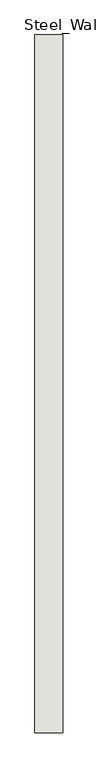
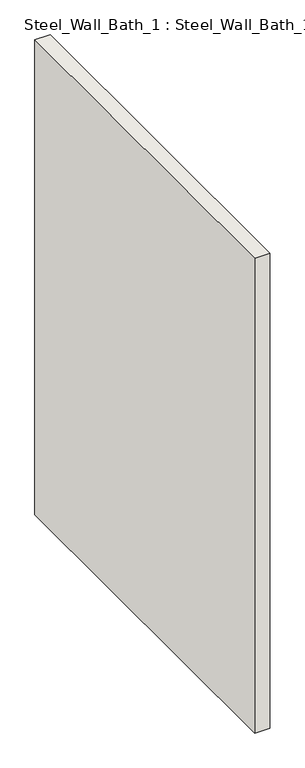
"""IFC4 building model written with IfcOpenShell, lengths in millimetres: wall geometry, Steel_Wall_Bath_1 : Steel_Wall_Bath_1."""

import ifcopenshell
import ifcopenshell.guid

model = None  # the IFC model being written
_history = None  # IfcOwnerHistory: only IFC2X3 demands one
_inside = {}  # id of a spatial element -> (the spatial element, [elements in it])
_under = {}  # id of a project, library or spatial element -> (it, [spatial elements below it])
_declared = {}  # id of a project -> (the project, [libraries it declares])
_typed = {}  # id of a type object -> (the type object, [elements of that type])
_made_of = {}  # id of a material, layer set ... -> (it, [elements and type objects made of it])


def new_model(schema):
    """Start an empty IFC model of exactly this schema.

    Asked for "IFC4X3", IfcOpenShell would pick the latest addendum, in which some entities
    have other attributes; the version numbers below select the first issue.
    IFC2X3 requires an IfcOwnerHistory on every rooted entity: one is made here for all.
    """
    global model, _history
    if schema == "IFC4X3":
        model = ifcopenshell.file(schema_version=(4, 3, 0, 0))
    else:
        model = ifcopenshell.file(schema=schema)
    _inside.clear()
    _under.clear()
    _declared.clear()
    _typed.clear()
    _made_of.clear()
    _history = None
    if model.schema == "IFC2X3":
        org = make("IfcOrganization", Name="unknown")
        user = make(
            "IfcPersonAndOrganization",
            ThePerson=make("IfcPerson", FamilyName="unknown"),
            TheOrganization=org,
        )
        app = make(
            "IfcApplication",
            ApplicationDeveloper=org,
            Version="unknown",
            ApplicationFullName="unknown",
            ApplicationIdentifier="unknown",
        )
        _history = make(
            "IfcOwnerHistory",
            OwningUser=user,
            OwningApplication=app,
            ChangeAction="ADDED",
            CreationDate=0,
        )
    return model


def make(cls, **values):
    """One entity of the class cls with the attributes given. An attribute that is None is left unset."""
    return model.create_entity(
        cls, **{name: value for name, value in values.items() if value is not None}
    )


def rooted(cls, **values):
    """An entity with a GlobalId (a new one), such as an element, a storey or a relation."""
    return make(cls, GlobalId=ifcopenshell.guid.new(), OwnerHistory=_history, **values)


def si_unit(unit_type, name, prefix=None):
    """IfcSIUnit, for example si_unit("LENGTHUNIT", "METRE", prefix="MILLI")."""
    return make("IfcSIUnit", UnitType=unit_type, Prefix=prefix, Name=name)


def assignment(units):
    """IfcUnitAssignment: the units of a project."""
    return None if units is None else make("IfcUnitAssignment", Units=units)


def point(xyz):
    """IfcCartesianPoint."""
    return None if xyz is None else make("IfcCartesianPoint", Coordinates=xyz)


def direction(xyz):
    """IfcDirection."""
    return None if xyz is None else make("IfcDirection", DirectionRatios=xyz)


def frame(location, z_axis=None, x_axis=None):
    """IfcAxis2Placement3D, a coordinate frame: its origin and axes. An axis left out is left unset."""
    return make(
        "IfcAxis2Placement3D",
        Location=point(location),
        Axis=direction(z_axis),
        RefDirection=direction(x_axis),
    )


def origin():
    """The frame at (0, 0, 0) with its axes left unset."""
    return frame((0.0, 0.0, 0.0))


def place(relative_to, where):
    """IfcLocalPlacement: puts the frame where relative to a parent placement (None: the world)."""
    return make(
        "IfcLocalPlacement", PlacementRelTo=relative_to, RelativePlacement=where
    )


def context(
    kind, dimensions, precision=None, world=None, true_north=None, identifier=None
):
    """IfcGeometricRepresentationContext, for example the 3D "Model" context."""
    return make(
        "IfcGeometricRepresentationContext",
        ContextIdentifier=identifier,
        ContextType=kind,
        CoordinateSpaceDimension=dimensions,
        Precision=precision,
        WorldCoordinateSystem=world,
        TrueNorth=true_north,
    )


def project(units=None, contexts=None):
    """IfcProject with its units and contexts."""
    return rooted(
        "IfcProject",
        Name="project",
        RepresentationContexts=contexts,
        UnitsInContext=assignment(units),
    )


def spatial(cls, under=None, at=None, **own):
    """A site, building, storey or space (cls), placed at a placement, below another one or the project."""
    s = rooted(cls, ObjectPlacement=at, **own)
    if under is not None:
        _under.setdefault(under.id(), (under, []))[1].append(s)
    return s


def polyline(points):
    """IfcPolyline through the points."""
    return make("IfcPolyline", Points=[point(p) for p in points])


def outline(outer, holes=None, kind="AREA"):
    """IfcArbitraryClosedProfileDef: a profile drawn as a closed curve; with holes, ...WithVoids."""
    if holes is None:
        return make("IfcArbitraryClosedProfileDef", ProfileType=kind, OuterCurve=outer)
    return make(
        "IfcArbitraryProfileDefWithVoids",
        ProfileType=kind,
        OuterCurve=outer,
        InnerCurves=holes,
    )


def extrude(swept, where, along, depth):
    """IfcExtrudedAreaSolid: the profile swept, set in the frame where, extruded along a direction by depth."""
    return make(
        "IfcExtrudedAreaSolid",
        SweptArea=swept,
        Position=where,
        ExtrudedDirection=direction(along),
        Depth=depth,
    )


def shape(context_of_items, identifier, shape_type, items):
    """IfcShapeRepresentation: the items that make up one representation, for example the "Body"."""
    return make(
        "IfcShapeRepresentation",
        ContextOfItems=context_of_items,
        RepresentationIdentifier=identifier,
        RepresentationType=shape_type,
        Items=items,
    )


def source(mapping_origin, context_of_items, identifier, shape_type, items):
    """IfcRepresentationMap: a shape defined once, which mapped items show again and again."""
    return make(
        "IfcRepresentationMap",
        MappingOrigin=mapping_origin,
        MappedRepresentation=shape(context_of_items, identifier, shape_type, items),
    )


def transform(
    local_origin,
    x_axis=None,
    y_axis=None,
    z_axis=None,
    scale=None,
    scale2=None,
    scale3=None,
    uniform=True,
):
    """IfcCartesianTransformationOperator3D, or its non-uniform kind. x_axis, y_axis, z_axis: its Axis1, 2, 3."""
    if uniform:
        return make(
            "IfcCartesianTransformationOperator3D",
            Axis1=direction(x_axis),
            Axis2=direction(y_axis),
            LocalOrigin=point(local_origin),
            Scale=scale,
            Axis3=direction(z_axis),
        )
    return make(
        "IfcCartesianTransformationOperator3DnonUniform",
        Axis1=direction(x_axis),
        Axis2=direction(y_axis),
        LocalOrigin=point(local_origin),
        Scale=scale,
        Axis3=direction(z_axis),
        Scale2=scale2,
        Scale3=scale3,
    )


def mapped(mapping_source, mapping_target):
    """IfcMappedItem: shows the shape of a source again, moved by a transform."""
    return make(
        "IfcMappedItem", MappingSource=mapping_source, MappingTarget=mapping_target
    )


def made_of(thing, what):
    """Note that an element or type object is made of a material, layer set ...; save() writes the relation."""
    if what is not None:
        _made_of.setdefault(what.id(), (what, []))[1].append(thing)
    return thing


def element(
    cls,
    number,
    at=None,
    inside=None,
    cuts=None,
    type_object=None,
    material=None,
    context=None,
    identifier="Body",
    shape_type=None,
    held_by="IfcProductDefinitionShape",
    body=None,
    shapes=None,
    **own,
):
    """One element of the class cls, such as IfcWall. Its Tag is "e" and its number.

    at: its placement. inside: the storey or other place that contains it. cuts: it is an
    opening in that element (IfcRelVoidsElement). A single representation is given by context,
    identifier, shape_type and body (its items); several are given by shapes. held_by: the class
    of the entity that holds the representations. save() writes the other relations.
    """
    e = rooted(cls, Tag="e%d" % number, ObjectPlacement=at, **own)
    if body is not None:
        shapes = [shape(context, identifier, shape_type, body)]
    if shapes is not None:
        e.Representation = make(held_by, Representations=shapes)
    if inside is not None:
        _inside.setdefault(inside.id(), (inside, []))[1].append(e)
    if cuts is not None:
        rooted(
            "IfcRelVoidsElement", RelatingBuildingElement=cuts, RelatedOpeningElement=e
        )
    if type_object is not None:
        _typed.setdefault(type_object.id(), (type_object, []))[1].append(e)
    return made_of(e, material)


def aggregate(whole, parts):
    """IfcRelAggregates: a whole, such as a stair, and the parts it consists of."""
    return rooted("IfcRelAggregates", RelatingObject=whole, RelatedObjects=parts)


def save(model, path):
    """Write the relations noted so far, then the file.

    IfcRelAggregates (storeys below a building ...), IfcRelContainedInSpatialStructure (elements
    in a storey), IfcRelDefinesByType, IfcRelAssociatesMaterial and IfcRelDeclares: one each for
    every whole, place, type object, material and project.
    """
    for whole, parts in _under.values():
        aggregate(whole, parts)
    for where, things in _inside.values():
        rooted(
            "IfcRelContainedInSpatialStructure",
            RelatedElements=things,
            RelatingStructure=where,
        )
    for kind, things in _typed.values():
        rooted("IfcRelDefinesByType", RelatedObjects=things, RelatingType=kind)
    for what, things in _made_of.values():
        rooted("IfcRelAssociatesMaterial", RelatedObjects=things, RelatingMaterial=what)
    for by, libraries in _declared.values():
        rooted("IfcRelDeclares", RelatingContext=by, RelatedDefinitions=libraries)
    model.write(path)


def steel_wall_bath_1_steel_wall_bath_1_50d80b11(model_context):
    return source(origin(), model_context, "Body", "SweptSolid", [
        extrude(outline(polyline([(4175.0, 14705.0), (4175.0, 12205.0), (4075.0, 12205.0), (4075.0, 14705.0), (4175.0, 14705.0)])), frame((0.0, 0.0, 250.0), z_axis=(0.0, 0.0, 1.0), x_axis=(1.0, 0.0, 0.0)), (0.0, 0.0, 1.0), 3300.0),
    ])


if __name__ == "__main__":
    model = new_model("IFC4")
    model_context = context("Model", 3, world=origin())
    ifc_project = project(units=[si_unit("LENGTHUNIT", "METRE", prefix="MILLI")], contexts=[model_context])
    site = spatial("IfcSite", under=ifc_project)
    building = spatial("IfcBuilding", under=site)
    placement = place(None, origin())
    steel_wall_bath_1_steel_wall_bath_1_shape = steel_wall_bath_1_steel_wall_bath_1_50d80b11(model_context)
    element("IfcWall", 1, ObjectType="Steel_Wall_Bath_1 : Steel_Wall_Bath_1", at=placement, inside=building, context=model_context, shape_type="MappedRepresentation", body=[
        mapped(steel_wall_bath_1_steel_wall_bath_1_shape, transform((0.0, 0.0, 0.0), x_axis=(1.0, 0.0, 0.0), y_axis=(0.0, 1.0, 0.0), z_axis=(0.0, 0.0, 1.0))),
    ])
    save(model, "model.ifc")

# Revit data of these elements
# Type "Steel_Wall_Bath_1 : Steel_Wall_Bath_1"
#   NameOverride = "Steel_Wall_Bath_1"
# Element 1 (IfcWall, "Steel_Wall_Bath_1 : Steel_Wall_Bath_1")
#   Materials on its faces: "IfcSurfaceStyle #33"
# Materials
#   "IfcSurfaceStyle #33": class "Unassigned", colour RGB 214 214 214, transparency 0
